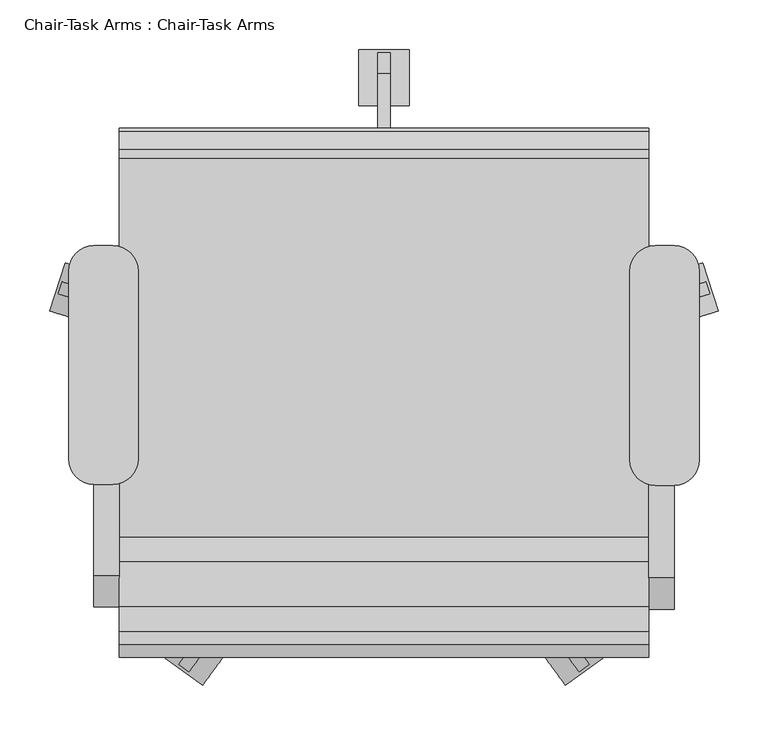
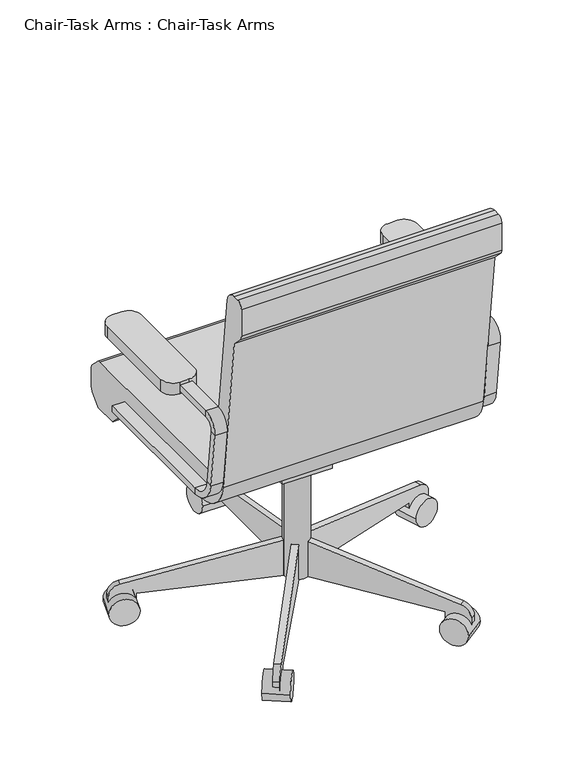
"""IFC4 building model written with IfcOpenShell, lengths in millimetres: furniture geometry, Chair-Task Arms : Chair-Task Arms."""

import ifcopenshell
import ifcopenshell.guid

model = None  # the IFC model being written
_history = None  # IfcOwnerHistory: only IFC2X3 demands one
_inside = {}  # id of a spatial element -> (the spatial element, [elements in it])
_under = {}  # id of a project, library or spatial element -> (it, [spatial elements below it])
_declared = {}  # id of a project -> (the project, [libraries it declares])
_typed = {}  # id of a type object -> (the type object, [elements of that type])
_made_of = {}  # id of a material, layer set ... -> (it, [elements and type objects made of it])


def new_model(schema):
    """Start an empty IFC model of exactly this schema.

    Asked for "IFC4X3", IfcOpenShell would pick the latest addendum, in which some entities
    have other attributes; the version numbers below select the first issue.
    IFC2X3 requires an IfcOwnerHistory on every rooted entity: one is made here for all.
    """
    global model, _history
    if schema == "IFC4X3":
        model = ifcopenshell.file(schema_version=(4, 3, 0, 0))
    else:
        model = ifcopenshell.file(schema=schema)
    _inside.clear()
    _under.clear()
    _declared.clear()
    _typed.clear()
    _made_of.clear()
    _history = None
    if model.schema == "IFC2X3":
        org = make("IfcOrganization", Name="unknown")
        user = make(
            "IfcPersonAndOrganization",
            ThePerson=make("IfcPerson", FamilyName="unknown"),
            TheOrganization=org,
        )
        app = make(
            "IfcApplication",
            ApplicationDeveloper=org,
            Version="unknown",
            ApplicationFullName="unknown",
            ApplicationIdentifier="unknown",
        )
        _history = make(
            "IfcOwnerHistory",
            OwningUser=user,
            OwningApplication=app,
            ChangeAction="ADDED",
            CreationDate=0,
        )
    return model


def make(cls, **values):
    """One entity of the class cls with the attributes given. An attribute that is None is left unset."""
    return model.create_entity(
        cls, **{name: value for name, value in values.items() if value is not None}
    )


def rooted(cls, **values):
    """An entity with a GlobalId (a new one), such as an element, a storey or a relation."""
    return make(cls, GlobalId=ifcopenshell.guid.new(), OwnerHistory=_history, **values)


def si_unit(unit_type, name, prefix=None):
    """IfcSIUnit, for example si_unit("LENGTHUNIT", "METRE", prefix="MILLI")."""
    return make("IfcSIUnit", UnitType=unit_type, Prefix=prefix, Name=name)


def assignment(units):
    """IfcUnitAssignment: the units of a project."""
    return None if units is None else make("IfcUnitAssignment", Units=units)


def point(xyz):
    """IfcCartesianPoint."""
    return None if xyz is None else make("IfcCartesianPoint", Coordinates=xyz)


def direction(xyz):
    """IfcDirection."""
    return None if xyz is None else make("IfcDirection", DirectionRatios=xyz)


def frame(location, z_axis=None, x_axis=None):
    """IfcAxis2Placement3D, a coordinate frame: its origin and axes. An axis left out is left unset."""
    return make(
        "IfcAxis2Placement3D",
        Location=point(location),
        Axis=direction(z_axis),
        RefDirection=direction(x_axis),
    )


def frame_2d(location, x_axis=None):
    """IfcAxis2Placement2D, a coordinate frame in the plane: its origin and x axis."""
    return make(
        "IfcAxis2Placement2D", Location=point(location), RefDirection=direction(x_axis)
    )


def origin():
    """The frame at (0, 0, 0) with its axes left unset."""
    return frame((0.0, 0.0, 0.0))


def place(relative_to, where):
    """IfcLocalPlacement: puts the frame where relative to a parent placement (None: the world)."""
    return make(
        "IfcLocalPlacement", PlacementRelTo=relative_to, RelativePlacement=where
    )


def context(
    kind, dimensions, precision=None, world=None, true_north=None, identifier=None
):
    """IfcGeometricRepresentationContext, for example the 3D "Model" context."""
    return make(
        "IfcGeometricRepresentationContext",
        ContextIdentifier=identifier,
        ContextType=kind,
        CoordinateSpaceDimension=dimensions,
        Precision=precision,
        WorldCoordinateSystem=world,
        TrueNorth=true_north,
    )


def project(units=None, contexts=None):
    """IfcProject with its units and contexts."""
    return rooted(
        "IfcProject",
        Name="project",
        RepresentationContexts=contexts,
        UnitsInContext=assignment(units),
    )


def spatial(cls, under=None, at=None, **own):
    """A site, building, storey or space (cls), placed at a placement, below another one or the project."""
    s = rooted(cls, ObjectPlacement=at, **own)
    if under is not None:
        _under.setdefault(under.id(), (under, []))[1].append(s)
    return s


def polyline(points):
    """IfcPolyline through the points."""
    return make("IfcPolyline", Points=[point(p) for p in points])


def circle_curve(where, radius):
    """IfcCircle in the frame where."""
    return make("IfcCircle", Position=where, Radius=radius)


def trimmed(basis, trim1, trim2, sense, master):
    """IfcTrimmedCurve: the piece of a basis curve between two trims."""
    return make(
        "IfcTrimmedCurve",
        BasisCurve=basis,
        Trim1=trim1,
        Trim2=trim2,
        SenseAgreement=sense,
        MasterRepresentation=master,
    )


def segment(curve, same_sense, transition):
    """IfcCompositeCurveSegment."""
    return make(
        "IfcCompositeCurveSegment",
        Transition=transition,
        SameSense=same_sense,
        ParentCurve=curve,
    )


def composite_curve(segments, self_intersect=None):
    """IfcCompositeCurve: segments joined end to end."""
    return make("IfcCompositeCurve", Segments=segments, SelfIntersect=self_intersect)


def outline(outer, holes=None, kind="AREA"):
    """IfcArbitraryClosedProfileDef: a profile drawn as a closed curve; with holes, ...WithVoids."""
    if holes is None:
        return make("IfcArbitraryClosedProfileDef", ProfileType=kind, OuterCurve=outer)
    return make(
        "IfcArbitraryProfileDefWithVoids",
        ProfileType=kind,
        OuterCurve=outer,
        InnerCurves=holes,
    )


def extrude(swept, where, along, depth):
    """IfcExtrudedAreaSolid: the profile swept, set in the frame where, extruded along a direction by depth."""
    return make(
        "IfcExtrudedAreaSolid",
        SweptArea=swept,
        Position=where,
        ExtrudedDirection=direction(along),
        Depth=depth,
    )


def shape(context_of_items, identifier, shape_type, items):
    """IfcShapeRepresentation: the items that make up one representation, for example the "Body"."""
    return make(
        "IfcShapeRepresentation",
        ContextOfItems=context_of_items,
        RepresentationIdentifier=identifier,
        RepresentationType=shape_type,
        Items=items,
    )


def source(mapping_origin, context_of_items, identifier, shape_type, items):
    """IfcRepresentationMap: a shape defined once, which mapped items show again and again."""
    return make(
        "IfcRepresentationMap",
        MappingOrigin=mapping_origin,
        MappedRepresentation=shape(context_of_items, identifier, shape_type, items),
    )


def transform(
    local_origin,
    x_axis=None,
    y_axis=None,
    z_axis=None,
    scale=None,
    scale2=None,
    scale3=None,
    uniform=True,
):
    """IfcCartesianTransformationOperator3D, or its non-uniform kind. x_axis, y_axis, z_axis: its Axis1, 2, 3."""
    if uniform:
        return make(
            "IfcCartesianTransformationOperator3D",
            Axis1=direction(x_axis),
            Axis2=direction(y_axis),
            LocalOrigin=point(local_origin),
            Scale=scale,
            Axis3=direction(z_axis),
        )
    return make(
        "IfcCartesianTransformationOperator3DnonUniform",
        Axis1=direction(x_axis),
        Axis2=direction(y_axis),
        LocalOrigin=point(local_origin),
        Scale=scale,
        Axis3=direction(z_axis),
        Scale2=scale2,
        Scale3=scale3,
    )


def mapped(mapping_source, mapping_target):
    """IfcMappedItem: shows the shape of a source again, moved by a transform."""
    return make(
        "IfcMappedItem", MappingSource=mapping_source, MappingTarget=mapping_target
    )


def made_of(thing, what):
    """Note that an element or type object is made of a material, layer set ...; save() writes the relation."""
    if what is not None:
        _made_of.setdefault(what.id(), (what, []))[1].append(thing)
    return thing


def element(
    cls,
    number,
    at=None,
    inside=None,
    cuts=None,
    type_object=None,
    material=None,
    context=None,
    identifier="Body",
    shape_type=None,
    held_by="IfcProductDefinitionShape",
    body=None,
    shapes=None,
    **own,
):
    """One element of the class cls, such as IfcWall. Its Tag is "e" and its number.

    at: its placement. inside: the storey or other place that contains it. cuts: it is an
    opening in that element (IfcRelVoidsElement). A single representation is given by context,
    identifier, shape_type and body (its items); several are given by shapes. held_by: the class
    of the entity that holds the representations. save() writes the other relations.
    """
    e = rooted(cls, Tag="e%d" % number, ObjectPlacement=at, **own)
    if body is not None:
        shapes = [shape(context, identifier, shape_type, body)]
    if shapes is not None:
        e.Representation = make(held_by, Representations=shapes)
    if inside is not None:
        _inside.setdefault(inside.id(), (inside, []))[1].append(e)
    if cuts is not None:
        rooted(
            "IfcRelVoidsElement", RelatingBuildingElement=cuts, RelatedOpeningElement=e
        )
    if type_object is not None:
        _typed.setdefault(type_object.id(), (type_object, []))[1].append(e)
    return made_of(e, material)


def aggregate(whole, parts):
    """IfcRelAggregates: a whole, such as a stair, and the parts it consists of."""
    return rooted("IfcRelAggregates", RelatingObject=whole, RelatedObjects=parts)


def save(model, path):
    """Write the relations noted so far, then the file.

    IfcRelAggregates (storeys below a building ...), IfcRelContainedInSpatialStructure (elements
    in a storey), IfcRelDefinesByType, IfcRelAssociatesMaterial and IfcRelDeclares: one each for
    every whole, place, type object, material and project.
    """
    for whole, parts in _under.values():
        aggregate(whole, parts)
    for where, things in _inside.values():
        rooted(
            "IfcRelContainedInSpatialStructure",
            RelatedElements=things,
            RelatingStructure=where,
        )
    for kind, things in _typed.values():
        rooted("IfcRelDefinesByType", RelatedObjects=things, RelatingType=kind)
    for what, things in _made_of.values():
        rooted("IfcRelAssociatesMaterial", RelatedObjects=things, RelatingMaterial=what)
    for by, libraries in _declared.values():
        rooted("IfcRelDeclares", RelatingContext=by, RelatedDefinitions=libraries)
    model.write(path)


def plane_surface(at):
    """IfcPlane: the flat surface through the origin of the frame at, square to its z axis."""
    return make("IfcPlane", Position=at)


def cylinder_surface(at, radius):
    """IfcCylindricalSurface: all points at the distance radius from the z axis of the frame at."""
    return make("IfcCylindricalSurface", Position=at, Radius=radius)


def revolved_surface(curve, axis_point, axis_direction):
    """IfcSurfaceOfRevolution: the curve turned about the line through axis_point along axis_direction."""
    return make(
        "IfcSurfaceOfRevolution",
        SweptCurve=make("IfcArbitraryOpenProfileDef", ProfileType="CURVE", Curve=curve),
        AxisPosition=make("IfcAxis1Placement", Location=point(axis_point), Axis=direction(axis_direction)),
    )


def advanced_brep(points, edges, surfaces, faces):
    """IfcAdvancedBrep: a solid bounded by faces that lie on surfaces and meet in shared edges.

    An edge is (start, end): straight between two places in points (the first is 0);
    or (start, end, curve); or (start, end, curve, False) where it runs against its curve.
    A face is (place in surfaces, loops), or (place, loops, False) where it looks against
    its surface's normal. A loop lists edges by number (the first is 1), with a minus sign
    where the edge is run from its end to its start. The first loop is the outer one.
    """
    corners = [point(p) for p in points]
    vertices = [make("IfcVertexPoint", VertexGeometry=c) for c in corners]
    made = []
    for start, end, *more in edges:
        made.append(
            make(
                "IfcEdgeCurve",
                EdgeStart=vertices[start],
                EdgeEnd=vertices[end],
                EdgeGeometry=more[0] if more else make("IfcPolyline", Points=[corners[start], corners[end]]),
                SameSense=more[1] if len(more) > 1 else True,
            )
        )
    hull = []
    for where, loops, *sense in faces:
        bounds = []
        for j, loop in enumerate(loops):
            ring = [make("IfcOrientedEdge", EdgeElement=made[abs(k) - 1], Orientation=k > 0) for k in loop]
            bounds.append(
                make(
                    "IfcFaceOuterBound" if j == 0 else "IfcFaceBound",
                    Bound=make("IfcEdgeLoop", EdgeList=ring),
                    Orientation=True,
                )
            )
        hull.append(make("IfcAdvancedFace", Bounds=bounds, FaceSurface=surfaces[where], SameSense=sense[0] if sense else True))
    return make("IfcAdvancedBrep", Outer=make("IfcClosedShell", CfsFaces=hull))


def chair_task_arms_chair_task_arms_8297d889(model_context):
    return source(origin(), model_context, "Body", "SolidModel", [
        extrude(outline(composite_curve([segment(polyline([(433.0908197, -74.2028048), (414.0408197, -74.2028048)]), True, "CONTINUOUS"), segment(trimmed(circle_curve(frame_2d((414.0408197, -48.8028048)), 25.4), [point((414.0408197, -74.2028048))], [point((388.6408197, -48.8028048))], False, "CARTESIAN"), True, "CONTINUOUS"), segment(polyline([(388.6408197, -48.8028048), (388.6408197, 141.6319091)]), True, "CONTINUOUS"), segment(trimmed(circle_curve(frame_2d((414.0408197, 141.6319091)), 25.4), [point((388.6408197, 141.6319091))], [point((414.0408197, 167.0319091))], False, "CARTESIAN"), True, "CONTINUOUS"), segment(polyline([(414.0408197, 167.0319091), (433.0908197, 167.0319091)]), True, "CONTINUOUS"), segment(trimmed(circle_curve(frame_2d((433.0908197, 141.6319091)), 25.4), [point((433.0908197, 167.0319091))], [point((458.4908197, 141.6319091))], False, "CARTESIAN"), True, "CONTINUOUS"), segment(polyline([(458.4908197, 141.6319091), (458.4908197, -48.8028048)]), True, "CONTINUOUS"), segment(trimmed(circle_curve(frame_2d((433.0908197, -48.8028048)), 25.4), [point((458.4908197, -48.8028048))], [point((433.0908197, -74.2028048))], False, "CARTESIAN"), True, "CONTINUOUS")], self_intersect=False)), frame((0.0, 0.0, 596.9), z_axis=(0.0, 0.0, 1.0), x_axis=(1.0, 0.0, 0.0)), (0.0, 0.0, 1.0), 25.4),
        extrude(outline(composite_curve([segment(polyline([(-132.0591803, -73.1575984), (-151.1091803, -73.1575984)]), True, "CONTINUOUS"), segment(trimmed(circle_curve(frame_2d((-151.1091803, -47.7575984)), 25.4), [point((-151.1091803, -73.1575984))], [point((-176.5091803, -47.7575984))], False, "CARTESIAN"), True, "CONTINUOUS"), segment(polyline([(-176.5091803, -47.7575984), (-176.5091803, 141.6319091)]), True, "CONTINUOUS"), segment(trimmed(circle_curve(frame_2d((-151.1091803, 141.6319091)), 25.4), [point((-176.5091803, 141.6319091))], [point((-151.1091803, 167.0319091))], False, "CARTESIAN"), True, "CONTINUOUS"), segment(polyline([(-151.1091803, 167.0319091), (-132.0591803, 167.0319091)]), True, "CONTINUOUS"), segment(trimmed(circle_curve(frame_2d((-132.0591803, 141.6319091)), 25.4), [point((-132.0591803, 167.0319091))], [point((-106.6591803, 141.6319091))], False, "CARTESIAN"), True, "CONTINUOUS"), segment(polyline([(-106.6591803, 141.6319091), (-106.6591803, -47.7575984)]), True, "CONTINUOUS"), segment(trimmed(circle_curve(frame_2d((-132.0591803, -47.7575984)), 25.4), [point((-106.6591803, -47.7575984))], [point((-132.0591803, -73.1575984))], False, "CARTESIAN"), True, "CONTINUOUS")], self_intersect=False)), frame((0.0, 0.0, 596.9), z_axis=(0.0, 0.0, 1.0), x_axis=(1.0, 0.0, 0.0)), (0.0, 0.0, 1.0), 25.4),
        advanced_brep(
        [(-151.1091803, 167.0319091, 412.75), (-151.1091803, 167.0319091, 425.45), (-125.7091803, 167.0319091, 425.45), (-125.7091803, 167.0319091, 412.75), (-151.1091803, -126.2388651, 412.75), (-151.1091803, -126.2388651, 425.45), (-125.7091803, -126.2388651, 425.45), (-125.7091803, -126.2388651, 412.75), (-151.1091803, -170.3844094, 464.7064065), (-151.1091803, -182.9974221, 463.2225227), (-125.7091803, -170.3844094, 464.7064065), (-125.7091803, -182.9974221, 463.2225227), (-151.1091803, -196.7936301, 580.4902904), (-151.1091803, -184.1806174, 581.9741742), (-125.7091803, -184.1806174, 581.9741742), (-125.7091803, -196.7936301, 580.4902904), (-151.1091803, -165.2610984, 603.25), (-151.1091803, -165.2610984, 615.95), (-125.7091803, -165.2610984, 603.25), (-125.7091803, -165.2610984, 615.95), (-151.1091803, 18.9459016, 615.95), (-125.7091803, 18.9459016, 615.95), (-125.7091803, 18.9459016, 603.25), (-151.1091803, 18.9459016, 603.25)],
        [
            (0, 1),
            (1, 2),
            (2, 3),
            (3, 0),
            (0, 4),
            (4, 5),
            (5, 1),
            (5, 6),
            (6, 2),
            (6, 7),
            (7, 3),
            (7, 4),
            (8, 5, circle_curve(frame((-151.1091803, -126.2388651, 469.9), z_axis=(1.0, 0.0, 0.0), x_axis=(0.0, 0.0, -1.0)), 44.45)),
            (4, 9, circle_curve(frame((-151.1091803, -126.2388651, 469.9), z_axis=(-1.0, 0.0, 0.0), x_axis=(0.0, 0.0, -1.0)), 57.15)),
            (9, 8),
            (10, 6, circle_curve(frame((-125.7091803, -126.2388651, 469.9), z_axis=(1.0, 0.0, 0.0), x_axis=(0.0, 0.0, -1.0)), 44.45)),
            (8, 10),
            (11, 7, circle_curve(frame((-125.7091803, -126.2388651, 469.9), z_axis=(1.0, 0.0, 0.0), x_axis=(0.0, 0.0, -1.0)), 57.15)),
            (10, 11),
            (11, 9),
            (9, 12),
            (12, 13),
            (13, 8),
            (13, 14),
            (14, 10),
            (14, 15),
            (15, 11),
            (15, 12),
            (16, 13, circle_curve(frame((-151.1091803, -165.2610984, 584.2), z_axis=(1.0, 0.0, 0.0), x_axis=(0.0, -0.993150604322877, -0.11684124756739026)), 19.05)),
            (12, 17, circle_curve(frame((-151.1091803, -165.2610984, 584.2), z_axis=(-1.0, 0.0, 0.0), x_axis=(0.0, -0.993150604322877, -0.11684124756739026)), 31.75)),
            (17, 16),
            (18, 14, circle_curve(frame((-125.7091803, -165.2610984, 584.2), z_axis=(1.0, 0.0, 0.0), x_axis=(0.0, -0.993150604322877, -0.11684124756739026)), 19.05)),
            (16, 18),
            (19, 15, circle_curve(frame((-125.7091803, -165.2610984, 584.2), z_axis=(1.0, 0.0, 0.0), x_axis=(0.0, -0.993150604322877, -0.11684124756739026)), 31.75)),
            (18, 19),
            (19, 17),
            (20, 21),
            (21, 22),
            (22, 23),
            (23, 20),
            (17, 20),
            (23, 16),
            (22, 18),
            (21, 19),
        ],
        [
            plane_surface(frame((-152.608212, 167.0319091, 419.1), z_axis=(0.0, 1.0, 0.0), x_axis=(0.0, 0.0, -1.0))),
            plane_surface(frame((-151.1091803, 167.0319091, 412.75), z_axis=(-1.0, 0.0, 0.0), x_axis=(0.0, -1.0, 0.0))),
            plane_surface(frame((-151.1091803, 167.0319091, 425.45), z_axis=(0.0, 0.0, 1.0), x_axis=(0.0, -1.0, 0.0))),
            plane_surface(frame((-125.7091803, 167.0319091, 425.45), z_axis=(1.0, 0.0, 0.0), x_axis=(0.0, -1.0, 0.0))),
            plane_surface(frame((-125.7091803, 167.0319091, 412.75), z_axis=(0.0, 0.0, -1.0), x_axis=(0.0, -1.0, 0.0))),
            plane_surface(frame((-151.1091803, -126.2388651, 469.9), z_axis=(-1.0, 0.0, 0.0), x_axis=(0.0, 0.0, -1.0))),
            revolved_surface(polyline([(-151.1091803, -126.2388651, 425.45), (-125.7091803, -126.2388651, 425.45)]), (-138.4091803, -126.2388651, 469.9), (-1.0, 0.0, 0.0)),
            plane_surface(frame((-125.7091803, -126.2388651, 469.9), z_axis=(1.0, 0.0, 0.0), x_axis=(0.0, 0.0, -1.0))),
            cylinder_surface(frame((-138.4091803, -126.2388651, 469.9), z_axis=(-1.0, 0.0, 0.0), x_axis=(0.0, 0.0, -1.0)), 57.15),
            plane_surface(frame((-151.1091803, -182.9974221, 463.2225227), z_axis=(-1.0, 0.0, 0.0), x_axis=(0.0, -0.11684124756738562, 0.9931506043228776))),
            plane_surface(frame((-151.1091803, -170.3844094, 464.7064065), z_axis=(0.0, 0.9931506043228776, 0.11684124756738562), x_axis=(0.0, -0.11684124756738562, 0.9931506043228776))),
            plane_surface(frame((-125.7091803, -170.3844094, 464.7064065), z_axis=(1.0, 0.0, 0.0), x_axis=(0.0, -0.11684124756738562, 0.9931506043228776))),
            plane_surface(frame((-125.7091803, -182.9974221, 463.2225227), z_axis=(0.0, -0.9931506043228776, -0.11684124756738562), x_axis=(0.0, -0.11684124756738562, 0.9931506043228776))),
            plane_surface(frame((-151.1091803, -165.2610984, 584.2), z_axis=(-1.0, 0.0, 0.0), x_axis=(0.0, -0.993150604322877, -0.11684124756739026))),
            revolved_surface(polyline([(-151.1091803, -184.1806174123508, 581.9741742338413), (-125.7091803, -184.1806174123508, 581.9741742338413)]), (-138.4091803, -165.2610984, 584.2), (-1.0, 0.0, 0.0)),
            plane_surface(frame((-125.7091803, -165.2610984, 584.2), z_axis=(1.0, 0.0, 0.0), x_axis=(0.0, -0.993150604322877, -0.11684124756739026))),
            cylinder_surface(frame((-138.4091803, -165.2610984, 584.2), z_axis=(-1.0, 0.0, 0.0), x_axis=(0.0, -0.993150604322877, -0.11684124756739026)), 31.75),
            plane_surface(frame((-152.608212, 18.9459016, 609.6), z_axis=(0.0, 1.0, 0.0), x_axis=(0.0, 0.0, 1.0))),
            plane_surface(frame((-151.1091803, -165.2610984, 615.95), z_axis=(-1.0, 0.0, 0.0), x_axis=(0.0, 1.0, 0.0))),
            plane_surface(frame((-151.1091803, -165.2610984, 603.25), z_axis=(0.0, 0.0, -1.0), x_axis=(0.0, 1.0, 0.0))),
            plane_surface(frame((-125.7091803, -165.2610984, 603.25), z_axis=(1.0, 0.0, 0.0), x_axis=(0.0, 1.0, 0.0))),
            plane_surface(frame((-125.7091803, -165.2610984, 615.95), z_axis=(0.0, 0.0, 1.0), x_axis=(0.0, 1.0, 0.0))),
        ],
        [
            (0, [[1, 2, 3, 4]]),
            (1, [[-1, 5, 6, 7]]),
            (2, [[-2, -7, 8, 9]]),
            (3, [[-3, -9, 10, 11]]),
            (4, [[-4, -11, 12, -5]]),
            (5, [[13, -6, 14, 15]]),
            (6, [[16, -8, -13, 17]]),
            (7, [[18, -10, -16, 19]]),
            (8, [[-14, -12, -18, 20]]),
            (9, [[-15, 21, 22, 23]]),
            (10, [[-17, -23, 24, 25]]),
            (11, [[-19, -25, 26, 27]]),
            (12, [[-20, -27, 28, -21]]),
            (13, [[29, -22, 30, 31]]),
            (14, [[32, -24, -29, 33]]),
            (15, [[34, -26, -32, 35]]),
            (16, [[-30, -28, -34, 36]]),
            (17, [[37, 38, 39, 40]]),
            (18, [[-31, 41, -40, 42]]),
            (19, [[-33, -42, -39, 43]]),
            (20, [[-35, -43, -38, 44]]),
            (21, [[-36, -44, -37, -41]]),
        ],
    ),
        advanced_brep(
        [(433.0908197, 167.0319091, 425.45), (433.0908197, 167.0319091, 412.75), (407.6908197, 167.0319091, 412.75), (407.6908197, 167.0319091, 425.45), (433.0908197, -128.329278, 425.45), (433.0908197, -128.329278, 412.75), (407.6908197, -128.329278, 412.75), (407.6908197, -128.329278, 425.45), (433.0908197, -185.0878351, 463.2225227), (433.0908197, -172.4748224, 464.7064065), (407.6908197, -185.0878351, 463.2225227), (407.6908197, -172.4748224, 464.7064065), (433.0908197, -186.2710303, 581.9741742), (433.0908197, -198.884043, 580.4902904), (407.6908197, -198.884043, 580.4902904), (407.6908197, -186.2710303, 581.9741742), (433.0908197, -167.3515113, 615.95), (433.0908197, -167.3515113, 603.25), (407.6908197, -167.3515113, 615.95), (407.6908197, -167.3515113, 603.25), (433.0908197, 18.9459016, 603.25), (407.6908197, 18.9459016, 603.25), (407.6908197, 18.9459016, 615.95), (433.0908197, 18.9459016, 615.95)],
        [
            (0, 1),
            (1, 2),
            (2, 3),
            (3, 0),
            (0, 4),
            (4, 5),
            (5, 1),
            (5, 6),
            (6, 2),
            (6, 7),
            (7, 3),
            (7, 4),
            (8, 5, circle_curve(frame((433.0908197, -128.329278, 469.9), z_axis=(1.0, 0.0, 0.0), x_axis=(0.0, 0.0, -1.0)), 57.15)),
            (4, 9, circle_curve(frame((433.0908197, -128.329278, 469.9), z_axis=(-1.0, 0.0, 0.0), x_axis=(0.0, 0.0, -1.0)), 44.45)),
            (9, 8),
            (10, 6, circle_curve(frame((407.6908197, -128.329278, 469.9), z_axis=(1.0, 0.0, 0.0), x_axis=(0.0, 0.0, -1.0)), 57.15)),
            (8, 10),
            (11, 7, circle_curve(frame((407.6908197, -128.329278, 469.9), z_axis=(1.0, 0.0, 0.0), x_axis=(0.0, 0.0, -1.0)), 44.45)),
            (10, 11),
            (11, 9),
            (9, 12),
            (12, 13),
            (13, 8),
            (13, 14),
            (14, 10),
            (14, 15),
            (15, 11),
            (15, 12),
            (16, 13, circle_curve(frame((433.0908197, -167.3515113, 584.2), z_axis=(1.0, 0.0, 0.0), x_axis=(0.0, -0.9931506043228767, -0.1168412475673929)), 31.75)),
            (12, 17, circle_curve(frame((433.0908197, -167.3515113, 584.2), z_axis=(-1.0, 0.0, 0.0), x_axis=(0.0, -0.9931506043228767, -0.1168412475673929)), 19.05)),
            (17, 16),
            (18, 14, circle_curve(frame((407.6908197, -167.3515113, 584.2), z_axis=(1.0, 0.0, 0.0), x_axis=(0.0, -0.9931506043228767, -0.1168412475673929)), 31.75)),
            (16, 18),
            (19, 15, circle_curve(frame((407.6908197, -167.3515113, 584.2), z_axis=(1.0, 0.0, 0.0), x_axis=(0.0, -0.9931506043228767, -0.1168412475673929)), 19.05)),
            (18, 19),
            (19, 17),
            (20, 21),
            (21, 22),
            (22, 23),
            (23, 20),
            (17, 20),
            (23, 16),
            (22, 18),
            (21, 19),
        ],
        [
            plane_surface(frame((406.191788, 167.0319091, 419.1), z_axis=(0.0, 1.0, 0.0), x_axis=(0.0, 0.0, -1.0))),
            plane_surface(frame((433.0908197, 167.0319091, 425.45), z_axis=(1.0, 0.0, 0.0), x_axis=(0.0, -1.0, 0.0))),
            plane_surface(frame((433.0908197, 167.0319091, 412.75), z_axis=(0.0, 0.0, -1.0), x_axis=(0.0, -1.0, 0.0))),
            plane_surface(frame((407.6908197, 167.0319091, 412.75), z_axis=(-1.0, 0.0, 0.0), x_axis=(0.0, -1.0, 0.0))),
            plane_surface(frame((407.6908197, 167.0319091, 425.45), z_axis=(0.0, 0.0, 1.0), x_axis=(0.0, -1.0, 0.0))),
            plane_surface(frame((433.0908197, -128.329278, 469.9), z_axis=(1.0, 0.0, 0.0), x_axis=(0.0, 0.0, -1.0))),
            cylinder_surface(frame((420.3908197, -128.329278, 469.9), z_axis=(-1.0, 0.0, 0.0), x_axis=(0.0, 0.0, -1.0)), 57.15),
            plane_surface(frame((407.6908197, -128.329278, 469.9), z_axis=(-1.0, 0.0, 0.0), x_axis=(0.0, 0.0, -1.0))),
            revolved_surface(polyline([(407.6908197, -128.329278, 425.45), (433.0908197, -128.329278, 425.45)]), (420.3908197, -128.329278, 469.9), (-1.0, 0.0, 0.0)),
            plane_surface(frame((433.0908197, -172.4748224, 464.7064065), z_axis=(1.0, 0.0, 0.0), x_axis=(0.0, -0.11684124756738622, 0.9931506043228775))),
            plane_surface(frame((433.0908197, -185.0878351, 463.2225227), z_axis=(0.0, -0.9931506043228775, -0.11684124756738622), x_axis=(0.0, -0.11684124756738622, 0.9931506043228775))),
            plane_surface(frame((407.6908197, -185.0878351, 463.2225227), z_axis=(-1.0, 0.0, 0.0), x_axis=(0.0, -0.11684124756738622, 0.9931506043228775))),
            plane_surface(frame((407.6908197, -172.4748224, 464.7064065), z_axis=(0.0, 0.9931506043228775, 0.11684124756738622), x_axis=(0.0, -0.11684124756738622, 0.9931506043228775))),
            plane_surface(frame((433.0908197, -167.3515113, 584.2), z_axis=(1.0, 0.0, 0.0), x_axis=(0.0, -0.9931506043228767, -0.1168412475673929))),
            cylinder_surface(frame((420.3908197, -167.3515113, 584.2), z_axis=(-1.0, 0.0, 0.0), x_axis=(0.0, -0.9931506043228767, -0.1168412475673929)), 31.75),
            plane_surface(frame((407.6908197, -167.3515113, 584.2), z_axis=(-1.0, 0.0, 0.0), x_axis=(0.0, -0.9931506043228767, -0.1168412475673929))),
            revolved_surface(polyline([(407.6908197, -186.2710303123508, 581.9741742338412), (433.0908197, -186.2710303123508, 581.9741742338412)]), (420.3908197, -167.3515113, 584.2), (-1.0, 0.0, 0.0)),
            plane_surface(frame((406.191788, 18.9459016, 609.6), z_axis=(0.0, 1.0, 0.0), x_axis=(0.0, 0.0, 1.0))),
            plane_surface(frame((433.0908197, -167.3515113, 603.25), z_axis=(1.0, 0.0, 0.0), x_axis=(0.0, 1.0, 0.0))),
            plane_surface(frame((433.0908197, -167.3515113, 615.95), z_axis=(0.0, 0.0, 1.0), x_axis=(0.0, 1.0, 0.0))),
            plane_surface(frame((407.6908197, -167.3515113, 615.95), z_axis=(-1.0, 0.0, 0.0), x_axis=(0.0, 1.0, 0.0))),
            plane_surface(frame((407.6908197, -167.3515113, 603.25), z_axis=(0.0, 0.0, -1.0), x_axis=(0.0, 1.0, 0.0))),
        ],
        [
            (0, [[1, 2, 3, 4]]),
            (1, [[-1, 5, 6, 7]]),
            (2, [[-2, -7, 8, 9]]),
            (3, [[-3, -9, 10, 11]]),
            (4, [[-4, -11, 12, -5]]),
            (5, [[13, -6, 14, 15]]),
            (6, [[16, -8, -13, 17]]),
            (7, [[18, -10, -16, 19]]),
            (8, [[-14, -12, -18, 20]]),
            (9, [[-15, 21, 22, 23]]),
            (10, [[-17, -23, 24, 25]]),
            (11, [[-19, -25, 26, 27]]),
            (12, [[-20, -27, 28, -21]]),
            (13, [[29, -22, 30, 31]]),
            (14, [[32, -24, -29, 33]]),
            (15, [[34, -26, -32, 35]]),
            (16, [[-30, -28, -34, 36]]),
            (17, [[37, 38, 39, 40]]),
            (18, [[-31, 41, -40, 42]]),
            (19, [[-33, -42, -39, 43]]),
            (20, [[-35, -43, -38, 44]]),
            (21, [[-36, -44, -37, -41]]),
        ],
    ),
        extrude(outline(composite_curve([segment(trimmed(circle_curve(frame_2d((140.9908197, 18.9459016)), 25.4), [point((115.5908197, 18.9459016))], [point((166.3908197, 18.9459016))], False, "CARTESIAN"), True, "CONTINUOUS"), segment(trimmed(circle_curve(frame_2d((140.9908197, 18.9459016)), 25.4), [point((166.3908197, 18.9459016))], [point((115.5908197, 18.9459016))], False, "CARTESIAN"), True, "CONTINUOUS")], self_intersect=False)), frame((0.0, 0.0, 53.5835944), z_axis=(0.0, 0.0, 1.0), x_axis=(1.0, 0.0, 0.0)), (0.0, 0.0, 1.0), 330.5914056),
        extrude(outline(composite_curve([segment(trimmed(circle_curve(frame_2d((0.0, -28.2002727)), 28.2002727), [point((0.0, -56.4005455))], [point((0.0, 0.0))], False, "CARTESIAN"), True, "CONTINUOUS"), segment(trimmed(circle_curve(frame_2d((0.0, -28.2002727)), 28.2002727), [point((0.0, 0.0))], [point((0.0, -56.4005455))], False, "CARTESIAN"), True, "CONTINUOUS")], self_intersect=False)), frame((477.6203484, 101.6163254, 28.1835944), z_axis=(-0.3090169943749423, 0.9510565162951553, 0.0), x_axis=(0.0, 0.0, 1.0)), (0.0, 0.0, 1.0), 50.8),
        extrude(outline(composite_curve([segment(polyline([(-25.4, 0.0), (0.0, 0.0), (0.0, -50.8), (-24.303053, -50.8)]), True, "CONTINUOUS"), segment(trimmed(circle_curve(frame_2d((-24.303053, -25.4)), 25.4), [point((-24.303053, -50.8))], [point((-49.3171699, -29.8106637))], False, "CARTESIAN"), True, "CONTINUOUS"), segment(polyline([(-49.3171699, -29.8106637), (-101.6, 266.7), (-101.6, 292.1), (-25.4, 292.1), (-25.4, 0.0)]), True, "CONTINUOUS")], self_intersect=False)), frame((420.756686, 103.1705568, 28.1835944), z_axis=(-0.3090169943749423, 0.9510565162951553, 0.0), x_axis=(0.0, 0.0, -1.0)), (0.0, 0.0, 1.0), 12.7),
        extrude(outline(composite_curve([segment(trimmed(circle_curve(frame_2d((0.0, -28.2002727)), 28.2002727), [point((0.0, -56.4005455))], [point((0.0, 0.0))], False, "CARTESIAN"), True, "CONTINUOUS"), segment(trimmed(circle_curve(frame_2d((0.0, -28.2002727)), 28.2002727), [point((0.0, 0.0))], [point((0.0, -56.4005455))], False, "CARTESIAN"), True, "CONTINUOUS")], self_intersect=False)), frame((323.63931, -275.6612394, 28.1835944), z_axis=(0.8090169943749499, 0.5877852522924699, 0.0), x_axis=(0.0, 0.0, 1.0)), (0.0, 0.0, 1.0), 50.8),
        extrude(outline(composite_curve([segment(polyline([(-25.4, 0.0), (0.0, 0.0), (0.0, -50.8), (-24.303053, -50.8)]), True, "CONTINUOUS"), segment(trimmed(circle_curve(frame_2d((-24.303053, -25.3999999)), 25.4), [point((-24.303053, -50.8))], [point((-49.3171699, -29.8106636))], False, "CARTESIAN"), True, "CONTINUOUS"), segment(polyline([(-49.3171699, -29.8106636), (-101.6, 266.7), (-101.6, 292.1), (-25.4, 292.1), (-25.4, 0.0)]), True, "CONTINUOUS")], self_intersect=False)), frame((307.545634, -221.1003988, 28.1835944), z_axis=(0.8090169943749499, 0.5877852522924699, 0.0), x_axis=(0.0, 0.0, -1.0)), (0.0, 0.0, 1.0), 12.7),
        extrude(outline(composite_curve([segment(trimmed(circle_curve(frame_2d((0.0, -28.2002727)), 28.2002727), [point((0.0, -56.4005455))], [point((0.0, 0.0))], False, "CARTESIAN"), True, "CONTINUOUS"), segment(trimmed(circle_curve(frame_2d((0.0, -28.2002727)), 28.2002727), [point((0.0, 0.0))], [point((0.0, -56.4005455))], False, "CARTESIAN"), True, "CONTINUOUS")], self_intersect=False)), frame((-41.6576707, -275.6612394, 28.1835944), z_axis=(-0.8090169943749458, 0.5877852522924754, 0.0), x_axis=(0.0, 0.0, -1.0)), (0.0, 0.0, 1.0), 50.8),
        extrude(outline(composite_curve([segment(polyline([(25.4, 0.0), (25.4, 292.1), (101.6, 292.1), (101.6, 266.7), (49.3171699, -29.8106637)]), True, "CONTINUOUS"), segment(trimmed(circle_curve(frame_2d((24.303053, -25.3999999)), 25.4), [point((49.3171699, -29.8106637))], [point((24.303053, -50.8))], False, "CARTESIAN"), True, "CONTINUOUS"), segment(polyline([(24.303053, -50.8), (0.0, -50.8), (0.0, 0.0), (25.4, 0.0)]), True, "CONTINUOUS")], self_intersect=False)), frame((-25.5639946, -221.1003988, 28.1835944), z_axis=(-0.8090169943749459, 0.5877852522924754, 0.0), x_axis=(0.0, 0.0, 1.0)), (0.0, 0.0, 1.0), 12.7),
        extrude(outline(composite_curve([segment(trimmed(circle_curve(frame_2d((0.0, -28.2002727)), 28.2002727), [point((0.0, -56.4005454))], [point((0.0, 0.0))], False, "CARTESIAN"), True, "CONTINUOUS"), segment(trimmed(circle_curve(frame_2d((0.0, -28.2002727)), 28.2002727), [point((0.0, 0.0))], [point((0.0, -56.4005454))], False, "CARTESIAN"), True, "CONTINUOUS")], self_intersect=False)), frame((-195.638709, 101.6163254, 28.1835944), z_axis=(0.3090169943749487, 0.9510565162951532, 0.0), x_axis=(0.0, 0.0, -1.0)), (0.0, 0.0, 1.0), 50.8),
        extrude(outline(composite_curve([segment(polyline([(25.4, 0.0), (25.4, 292.1000001), (101.6, 292.1000001), (101.6, 266.7), (49.3171699, -29.8106636)]), True, "CONTINUOUS"), segment(trimmed(circle_curve(frame_2d((24.303053, -25.4)), 25.4), [point((49.3171699, -29.8106636))], [point((24.303053, -50.8))], False, "CARTESIAN"), True, "CONTINUOUS"), segment(polyline([(24.303053, -50.8), (0.0, -50.8), (0.0, 0.0), (25.4, 0.0)]), True, "CONTINUOUS")], self_intersect=False)), frame((-138.7750467, 103.1705568, 28.1835944), z_axis=(0.3090169943749487, 0.9510565162951532, 0.0), x_axis=(0.0, 0.0, 1.0)), (0.0, 0.0, 1.0), 12.7),
        extrude(outline(composite_curve([segment(trimmed(circle_curve(frame_2d((336.4459016, 28.1835944)), 28.2002727), [point((308.2456289, 28.1835944))], [point((364.6461744, 28.1835944))], False, "CARTESIAN"), True, "CONTINUOUS"), segment(trimmed(circle_curve(frame_2d((336.4459016, 28.1835944)), 28.2002727), [point((364.6461744, 28.1835944))], [point((308.2456289, 28.1835944))], False, "CARTESIAN"), True, "CONTINUOUS")], self_intersect=False)), frame((115.5908197, 0.0, 0.0), z_axis=(1.0, 0.0, 0.0), x_axis=(0.0, 1.0, 0.0)), (0.0, 0.0, 1.0), 50.8),
        extrude(outline(composite_curve([segment(polyline([(311.0459016, 53.5835944), (18.9459016, 53.5835944), (18.9459016, 129.7835944), (44.3459016, 129.7835944), (340.8565654, 77.5007643)]), True, "CONTINUOUS"), segment(trimmed(circle_curve(frame_2d((336.4459016, 52.4866474)), 25.4), [point((340.8565654, 77.5007643))], [point((361.8459016, 52.4866474))], False, "CARTESIAN"), True, "CONTINUOUS"), segment(polyline([(361.8459016, 52.4866474), (361.8459016, 28.1835944), (311.0459016, 28.1835944), (311.0459016, 53.5835944)]), True, "CONTINUOUS")], self_intersect=False)), frame((134.6408197, 0.0, 0.0), z_axis=(1.0, 0.0, 0.0), x_axis=(0.0, 1.0, 0.0)), (0.0, 0.0, 1.0), 12.7),
        extrude(outline(polyline([(69.7459016, 383.7835944), (69.7459016, 371.0835944), (18.9459016, 283.0954134), (-19.1540984, 283.0954134), (-19.1540984, 383.7835944), (69.7459016, 383.7835944)])), frame((90.1908197, 0.0, 0.0), z_axis=(1.0, 0.0, 0.0), x_axis=(0.0, 1.0, 0.0)), (0.0, 0.0, 1.0), 101.6),
        extrude(outline(composite_curve([segment(polyline([(-126.2050455, 457.2), (255.0102301, 457.2)]), True, "CONTINUOUS"), segment(trimmed(circle_curve(frame_2d((255.0102301, 444.5)), 12.7), [point((255.0102301, 457.2))], [point((263.9604301, 453.510212))], False, "CARTESIAN"), True, "CONTINUOUS"), segment(polyline([(263.9604301, 453.510212), (281.8961016, 435.6939999)]), True, "CONTINUOUS"), segment(trimmed(circle_curve(frame_2d((272.9459016, 426.6837879)), 12.7), [point((281.8961016, 435.6939999))], [point((285.6459016, 426.6837879))], False, "CARTESIAN"), True, "CONTINUOUS"), segment(polyline([(285.6459016, 426.6837879), (285.6459016, 391.6405184)]), True, "CONTINUOUS"), segment(trimmed(circle_curve(frame_2d((260.2459016, 391.6405184)), 25.4), [point((285.6459016, 391.6405184))], [point((278.2663256, 373.7401184))], False, "CARTESIAN"), True, "CONTINUOUS"), segment(polyline([(278.2663256, 373.7401184), (260.2470284, 355.6), (209.4470284, 355.6), (181.0744602, 383.7835944), (-107.1089978, 383.7835944)]), True, "CONTINUOUS"), segment(trimmed(circle_curve(frame_2d((-107.1089978, 459.9835944)), 76.2), [point((-107.1089978, 383.7835944))], [point((-182.7870738, 451.0802913))], False, "CARTESIAN"), True, "CONTINUOUS"), segment(polyline([(-182.7870738, 451.0802913), (-222.3540984, 787.4), (-244.0343545, 809.0802561)]), True, "CONTINUOUS"), segment(trimmed(circle_curve(frame_2d((-235.0540984, 818.0605122)), 12.7), [point((-244.0343545, 809.0802561))], [point((-247.7540984, 818.0605122))], False, "CARTESIAN"), True, "CONTINUOUS"), segment(polyline([(-247.7540984, 818.0605122), (-247.7540984, 876.3)]), True, "CONTINUOUS"), segment(trimmed(circle_curve(frame_2d((-235.0540984, 876.3)), 12.7), [point((-247.7540984, 876.3))], [point((-235.0540984, 889.0))], False, "CARTESIAN"), True, "CONTINUOUS"), segment(polyline([(-235.0540984, 889.0), (-222.1789239, 889.0)]), True, "CONTINUOUS"), segment(trimmed(circle_curve(frame_2d((-222.1789239, 863.6)), 25.4), [point((-222.1789239, 889.0))], [point((-196.9528985, 866.5677677))], False, "CARTESIAN"), True, "CONTINUOUS"), segment(polyline([(-196.9528985, 866.5677677), (-151.4310708, 479.6322323)]), True, "CONTINUOUS"), segment(trimmed(circle_curve(frame_2d((-126.2050455, 482.6)), 25.4), [point((-151.4310708, 479.6322323))], [point((-126.2050455, 457.2))], True, "CARTESIAN"), True, "CONTINUOUS")], self_intersect=False)), frame((-125.7091803, 0.0, 0.0), z_axis=(1.0, 0.0, 0.0), x_axis=(0.0, 1.0, 0.0)), (0.0, 0.0, 1.0), 533.4),
    ])


if __name__ == "__main__":
    model = new_model("IFC4")
    model_context = context("Model", 3, world=origin())
    ifc_project = project(units=[si_unit("LENGTHUNIT", "METRE", prefix="MILLI")], contexts=[model_context])
    site = spatial("IfcSite", under=ifc_project)
    building = spatial("IfcBuilding", under=site)
    placement = place(None, origin())
    chair_task_arms_chair_task_arms_shape = chair_task_arms_chair_task_arms_8297d889(model_context)
    element("IfcFurniture", 1, ObjectType="Chair-Task Arms : Chair-Task Arms", at=placement, inside=building, context=model_context, shape_type="MappedRepresentation", body=[
        mapped(chair_task_arms_chair_task_arms_shape, transform((0.0, 0.0, 0.0), x_axis=(1.0, 0.0, 0.0), y_axis=(0.0, 1.0, 0.0), z_axis=(0.0, 0.0, 1.0))),
    ])
    save(model, "model.ifc")

# Revit data of these elements
# Type "Chair-Task Arms : Chair-Task Arms"
#   Model = "CHTSK-095"
#   Manufacturer = "Furniture Concepts"
#   Type Mark = "CH-3"
#   Assembly Code = "E2020200"
#   Cost = 1095
#   Base Material = Plastic, Opaque Black
#   Caster Material = Plastic, Opaque Black
#   Seat/Back Material = Leather - Matte (Tan)
#   Default Elevation = 0
# Element 1 (IfcFurniture, "Chair-Task Arms : Chair-Task Arms")
#   Materials on its faces: "Plastic, Opaque Black", "Leather - Matte (Tan)"
# Materials
#   "Plastic, Opaque Black": class "Plastic", colour RGB 0 0 0, transparency 0, Description = "Plastic, generic, opaque black", Cost = 0
#   "Leather - Matte (Tan)": class "Generic", colour RGB 162 130 69, transparency 0, Cost = 0
